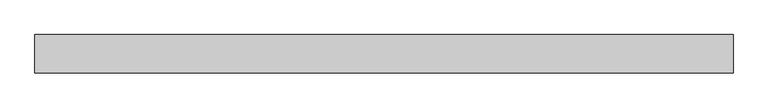
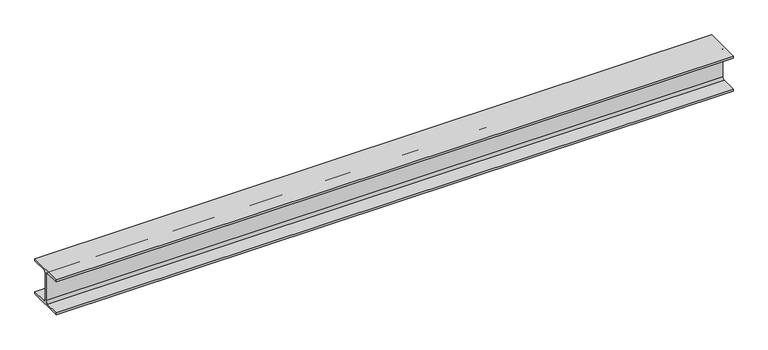
"""IFC4 building model written with IfcOpenShell, lengths in millimetres: beam geometry, 0912_Steel Framing_H-KSD3502 : H_SB_ASB_H-200x200x8x12."""

import ifcopenshell
import ifcopenshell.guid

model = None  # the IFC model being written
_history = None  # IfcOwnerHistory: only IFC2X3 demands one
_inside = {}  # id of a spatial element -> (the spatial element, [elements in it])
_under = {}  # id of a project, library or spatial element -> (it, [spatial elements below it])
_declared = {}  # id of a project -> (the project, [libraries it declares])
_typed = {}  # id of a type object -> (the type object, [elements of that type])
_made_of = {}  # id of a material, layer set ... -> (it, [elements and type objects made of it])


def new_model(schema):
    """Start an empty IFC model of exactly this schema.

    Asked for "IFC4X3", IfcOpenShell would pick the latest addendum, in which some entities
    have other attributes; the version numbers below select the first issue.
    IFC2X3 requires an IfcOwnerHistory on every rooted entity: one is made here for all.
    """
    global model, _history
    if schema == "IFC4X3":
        model = ifcopenshell.file(schema_version=(4, 3, 0, 0))
    else:
        model = ifcopenshell.file(schema=schema)
    _inside.clear()
    _under.clear()
    _declared.clear()
    _typed.clear()
    _made_of.clear()
    _history = None
    if model.schema == "IFC2X3":
        org = make("IfcOrganization", Name="unknown")
        user = make(
            "IfcPersonAndOrganization",
            ThePerson=make("IfcPerson", FamilyName="unknown"),
            TheOrganization=org,
        )
        app = make(
            "IfcApplication",
            ApplicationDeveloper=org,
            Version="unknown",
            ApplicationFullName="unknown",
            ApplicationIdentifier="unknown",
        )
        _history = make(
            "IfcOwnerHistory",
            OwningUser=user,
            OwningApplication=app,
            ChangeAction="ADDED",
            CreationDate=0,
        )
    return model


def make(cls, **values):
    """One entity of the class cls with the attributes given. An attribute that is None is left unset."""
    return model.create_entity(
        cls, **{name: value for name, value in values.items() if value is not None}
    )


def rooted(cls, **values):
    """An entity with a GlobalId (a new one), such as an element, a storey or a relation."""
    return make(cls, GlobalId=ifcopenshell.guid.new(), OwnerHistory=_history, **values)


def si_unit(unit_type, name, prefix=None):
    """IfcSIUnit, for example si_unit("LENGTHUNIT", "METRE", prefix="MILLI")."""
    return make("IfcSIUnit", UnitType=unit_type, Prefix=prefix, Name=name)


def assignment(units):
    """IfcUnitAssignment: the units of a project."""
    return None if units is None else make("IfcUnitAssignment", Units=units)


def point(xyz):
    """IfcCartesianPoint."""
    return None if xyz is None else make("IfcCartesianPoint", Coordinates=xyz)


def direction(xyz):
    """IfcDirection."""
    return None if xyz is None else make("IfcDirection", DirectionRatios=xyz)


def frame(location, z_axis=None, x_axis=None):
    """IfcAxis2Placement3D, a coordinate frame: its origin and axes. An axis left out is left unset."""
    return make(
        "IfcAxis2Placement3D",
        Location=point(location),
        Axis=direction(z_axis),
        RefDirection=direction(x_axis),
    )


def frame_2d(location, x_axis=None):
    """IfcAxis2Placement2D, a coordinate frame in the plane: its origin and x axis."""
    return make(
        "IfcAxis2Placement2D", Location=point(location), RefDirection=direction(x_axis)
    )


def origin():
    """The frame at (0, 0, 0) with its axes left unset."""
    return frame((0.0, 0.0, 0.0))


def place(relative_to, where):
    """IfcLocalPlacement: puts the frame where relative to a parent placement (None: the world)."""
    return make(
        "IfcLocalPlacement", PlacementRelTo=relative_to, RelativePlacement=where
    )


def context(
    kind, dimensions, precision=None, world=None, true_north=None, identifier=None
):
    """IfcGeometricRepresentationContext, for example the 3D "Model" context."""
    return make(
        "IfcGeometricRepresentationContext",
        ContextIdentifier=identifier,
        ContextType=kind,
        CoordinateSpaceDimension=dimensions,
        Precision=precision,
        WorldCoordinateSystem=world,
        TrueNorth=true_north,
    )


def project(units=None, contexts=None):
    """IfcProject with its units and contexts."""
    return rooted(
        "IfcProject",
        Name="project",
        RepresentationContexts=contexts,
        UnitsInContext=assignment(units),
    )


def spatial(cls, under=None, at=None, **own):
    """A site, building, storey or space (cls), placed at a placement, below another one or the project."""
    s = rooted(cls, ObjectPlacement=at, **own)
    if under is not None:
        _under.setdefault(under.id(), (under, []))[1].append(s)
    return s


def polyline(points):
    """IfcPolyline through the points."""
    return make("IfcPolyline", Points=[point(p) for p in points])


def circle_curve(where, radius):
    """IfcCircle in the frame where."""
    return make("IfcCircle", Position=where, Radius=radius)


def trimmed(basis, trim1, trim2, sense, master):
    """IfcTrimmedCurve: the piece of a basis curve between two trims."""
    return make(
        "IfcTrimmedCurve",
        BasisCurve=basis,
        Trim1=trim1,
        Trim2=trim2,
        SenseAgreement=sense,
        MasterRepresentation=master,
    )


def segment(curve, same_sense, transition):
    """IfcCompositeCurveSegment."""
    return make(
        "IfcCompositeCurveSegment",
        Transition=transition,
        SameSense=same_sense,
        ParentCurve=curve,
    )


def composite_curve(segments, self_intersect=None):
    """IfcCompositeCurve: segments joined end to end."""
    return make("IfcCompositeCurve", Segments=segments, SelfIntersect=self_intersect)


def outline(outer, holes=None, kind="AREA"):
    """IfcArbitraryClosedProfileDef: a profile drawn as a closed curve; with holes, ...WithVoids."""
    if holes is None:
        return make("IfcArbitraryClosedProfileDef", ProfileType=kind, OuterCurve=outer)
    return make(
        "IfcArbitraryProfileDefWithVoids",
        ProfileType=kind,
        OuterCurve=outer,
        InnerCurves=holes,
    )


def extrude(swept, where, along, depth):
    """IfcExtrudedAreaSolid: the profile swept, set in the frame where, extruded along a direction by depth."""
    return make(
        "IfcExtrudedAreaSolid",
        SweptArea=swept,
        Position=where,
        ExtrudedDirection=direction(along),
        Depth=depth,
    )


def shape(context_of_items, identifier, shape_type, items):
    """IfcShapeRepresentation: the items that make up one representation, for example the "Body"."""
    return make(
        "IfcShapeRepresentation",
        ContextOfItems=context_of_items,
        RepresentationIdentifier=identifier,
        RepresentationType=shape_type,
        Items=items,
    )


def source(mapping_origin, context_of_items, identifier, shape_type, items):
    """IfcRepresentationMap: a shape defined once, which mapped items show again and again."""
    return make(
        "IfcRepresentationMap",
        MappingOrigin=mapping_origin,
        MappedRepresentation=shape(context_of_items, identifier, shape_type, items),
    )


def transform(
    local_origin,
    x_axis=None,
    y_axis=None,
    z_axis=None,
    scale=None,
    scale2=None,
    scale3=None,
    uniform=True,
):
    """IfcCartesianTransformationOperator3D, or its non-uniform kind. x_axis, y_axis, z_axis: its Axis1, 2, 3."""
    if uniform:
        return make(
            "IfcCartesianTransformationOperator3D",
            Axis1=direction(x_axis),
            Axis2=direction(y_axis),
            LocalOrigin=point(local_origin),
            Scale=scale,
            Axis3=direction(z_axis),
        )
    return make(
        "IfcCartesianTransformationOperator3DnonUniform",
        Axis1=direction(x_axis),
        Axis2=direction(y_axis),
        LocalOrigin=point(local_origin),
        Scale=scale,
        Axis3=direction(z_axis),
        Scale2=scale2,
        Scale3=scale3,
    )


def mapped(mapping_source, mapping_target):
    """IfcMappedItem: shows the shape of a source again, moved by a transform."""
    return make(
        "IfcMappedItem", MappingSource=mapping_source, MappingTarget=mapping_target
    )


def made_of(thing, what):
    """Note that an element or type object is made of a material, layer set ...; save() writes the relation."""
    if what is not None:
        _made_of.setdefault(what.id(), (what, []))[1].append(thing)
    return thing


def element(
    cls,
    number,
    at=None,
    inside=None,
    cuts=None,
    type_object=None,
    material=None,
    context=None,
    identifier="Body",
    shape_type=None,
    held_by="IfcProductDefinitionShape",
    body=None,
    shapes=None,
    **own,
):
    """One element of the class cls, such as IfcWall. Its Tag is "e" and its number.

    at: its placement. inside: the storey or other place that contains it. cuts: it is an
    opening in that element (IfcRelVoidsElement). A single representation is given by context,
    identifier, shape_type and body (its items); several are given by shapes. held_by: the class
    of the entity that holds the representations. save() writes the other relations.
    """
    e = rooted(cls, Tag="e%d" % number, ObjectPlacement=at, **own)
    if body is not None:
        shapes = [shape(context, identifier, shape_type, body)]
    if shapes is not None:
        e.Representation = make(held_by, Representations=shapes)
    if inside is not None:
        _inside.setdefault(inside.id(), (inside, []))[1].append(e)
    if cuts is not None:
        rooted(
            "IfcRelVoidsElement", RelatingBuildingElement=cuts, RelatedOpeningElement=e
        )
    if type_object is not None:
        _typed.setdefault(type_object.id(), (type_object, []))[1].append(e)
    return made_of(e, material)


def aggregate(whole, parts):
    """IfcRelAggregates: a whole, such as a stair, and the parts it consists of."""
    return rooted("IfcRelAggregates", RelatingObject=whole, RelatedObjects=parts)


def save(model, path):
    """Write the relations noted so far, then the file.

    IfcRelAggregates (storeys below a building ...), IfcRelContainedInSpatialStructure (elements
    in a storey), IfcRelDefinesByType, IfcRelAssociatesMaterial and IfcRelDeclares: one each for
    every whole, place, type object, material and project.
    """
    for whole, parts in _under.values():
        aggregate(whole, parts)
    for where, things in _inside.values():
        rooted(
            "IfcRelContainedInSpatialStructure",
            RelatedElements=things,
            RelatingStructure=where,
        )
    for kind, things in _typed.values():
        rooted("IfcRelDefinesByType", RelatedObjects=things, RelatingType=kind)
    for what, things in _made_of.values():
        rooted("IfcRelAssociatesMaterial", RelatedObjects=things, RelatingMaterial=what)
    for by, libraries in _declared.values():
        rooted("IfcRelDeclares", RelatingContext=by, RelatedDefinitions=libraries)
    model.write(path)


def beam_3ecbfdb4(model_context):
    return source(origin(), model_context, "Body", "SweptSolid", [
        extrude(outline(composite_curve([segment(polyline([(100.0, -88.0), (100.0, -100.0), (-100.0, -100.0), (-100.0, -88.0), (-17.0, -88.0)]), True, "CONTINUOUS"), segment(trimmed(circle_curve(frame_2d((-17.0, -75.0)), 13.0), [point((-17.0, -88.0))], [point((-4.0, -75.0))], True, "CARTESIAN"), True, "CONTINUOUS"), segment(polyline([(-4.0, -75.0), (-4.0, 75.0)]), True, "CONTINUOUS"), segment(trimmed(circle_curve(frame_2d((-17.0, 75.0)), 13.0), [point((-4.0, 75.0))], [point((-17.0, 88.0))], True, "CARTESIAN"), True, "CONTINUOUS"), segment(polyline([(-17.0, 88.0), (-100.0, 88.0), (-100.0, 100.0), (100.0, 100.0), (100.0, 88.0), (17.0, 88.0)]), True, "CONTINUOUS"), segment(trimmed(circle_curve(frame_2d((17.0, 75.0)), 13.0), [point((17.0, 88.0))], [point((4.0, 75.0))], True, "CARTESIAN"), True, "CONTINUOUS"), segment(polyline([(4.0, 75.0), (4.0, -75.0)]), True, "CONTINUOUS"), segment(trimmed(circle_curve(frame_2d((17.0, -75.0)), 13.0), [point((4.0, -75.0))], [point((17.0, -88.0))], True, "CARTESIAN"), True, "CONTINUOUS"), segment(polyline([(17.0, -88.0), (100.0, -88.0)]), True, "CONTINUOUS")], self_intersect=False)), frame((-1914.9296967, 0.0, 0.0), z_axis=(1.0, 0.0, 0.0), x_axis=(0.0, 1.0, 0.0)), (0.0, 0.0, 1.0), 3642.6434861),
    ])


if __name__ == "__main__":
    model = new_model("IFC4")
    model_context = context("Model", 3, world=origin())
    ifc_project = project(units=[si_unit("LENGTHUNIT", "METRE", prefix="MILLI")], contexts=[model_context])
    site = spatial("IfcSite", under=ifc_project)
    building = spatial("IfcBuilding", under=site)
    placement = place(None, origin())
    beam_shape = beam_3ecbfdb4(model_context)
    element("IfcBeam", 1, ObjectType="0912_Steel Framing_H-KSD3502 : H_SB_ASB_H-200x200x8x12", at=placement, inside=building, context=model_context, shape_type="MappedRepresentation", body=[
        mapped(beam_shape, transform((0.0, 0.0, 0.0), x_axis=(1.0, 0.0, 0.0), y_axis=(0.0, 1.0, 0.0), z_axis=(0.0, 0.0, 1.0))),
    ])
    save(model, "model.ifc")

# Revit data of these elements
# Type "0912_Steel Framing_H-KSD3502 : H_SB_ASB_H-200x200x8x12"
#   H_WM Code_1 = "S01AA002-00001 | Main Steel Structure Fabrication Work | Shelter/Building | Medium Steel - Standard (90KG/M>Weight≥30KG/M) | Material: (   )"
#   H_WM Code_2 = "S03AA028-00001 | Main Steel Structure Erection Work | Shelter/Building | Medium Steel (90KG/M>Weight≥30KG/M) | Material: (   )"
#   H_WM Code_3 = "S01AA010-00001 | Main Steel Structure Fabrication Work | Shelter/Building | Steel Painting/Coating | for Non-Fireproofed Steel Surface, Surface Preparation, Primer, Second & Final Coat | Material: (   )"
#   H_Q'ty Cal Type Tag = "SB-Q2"
#   Width = 20.0 cm
#   Web Thickness = 0.8 cm
#   Web Fillet = 1.3 cm
#   Warping Constant = 141000.0 cm⁶
#   W = 0
#   Torsional Moment of Inertia = 26.2485 cm⁴
#   Section Area = 63.53 cm²
#   Plastic Modulus weak axis = 244.0 cm³
#   Plastic Modulus strong axis = 525.0 cm³
#   Perimeter = 1.16 m²/m
#   Nominal Weight = 49.90 kgf/m
#   Moment of Inertia weak axis = 1600.00 cm⁴
#   Moment of Inertia strong axis = 4720.00 cm⁴
#   Height = 20.0 cm
#   Flange Thickness = 1.2 cm
#   Elastic Modulus weak axis = 160.0 cm³
#   Elastic Modulus strong axis = 472.0 cm³
#   Centroid Vertical = 10.0 cm
#   Centroid Horizontal = 10.0 cm
#   Ix = 47200000
#   Length [instance default] = 1.5240 m
#   Zx = 525000
#   b = 0.2000 m
#   h = 0.2000 m
#   r = 0.0130 m
#   s = 0.0080 m
#   t = 0.0120 m
#   A = 0.006353 m²
#   Structural Material [instance default] = Steel, 45-345
#   Assembly Code = ""
# Element 1 (IfcBeam, "0912_Steel Framing_H-KSD3502 : H_SB_ASB_H-200x200x8x12")
#   Structural Material = none
# Materials
#   "Steel, 45-345": class "Metal", colour RGB 189 187 185, transparency 0, Description = "Steel 345 MPa", Cost = 0
